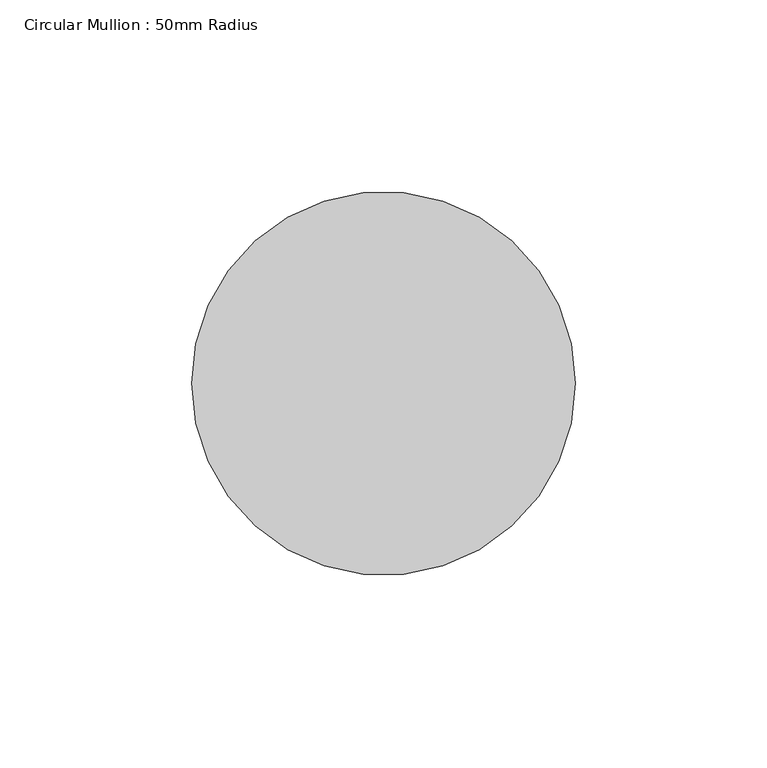
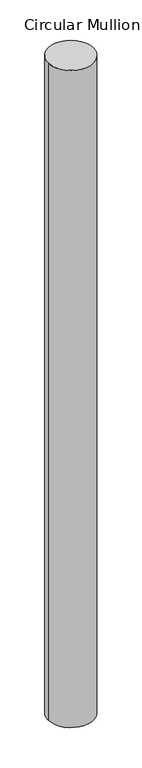
"""IFC4 building model written with IfcOpenShell, lengths in millimetres: member geometry, Circular Mullion : 50mm Radius."""

import ifcopenshell
import ifcopenshell.guid

model = None  # the IFC model being written
_history = None  # IfcOwnerHistory: only IFC2X3 demands one
_inside = {}  # id of a spatial element -> (the spatial element, [elements in it])
_under = {}  # id of a project, library or spatial element -> (it, [spatial elements below it])
_declared = {}  # id of a project -> (the project, [libraries it declares])
_typed = {}  # id of a type object -> (the type object, [elements of that type])
_made_of = {}  # id of a material, layer set ... -> (it, [elements and type objects made of it])


def new_model(schema):
    """Start an empty IFC model of exactly this schema.

    Asked for "IFC4X3", IfcOpenShell would pick the latest addendum, in which some entities
    have other attributes; the version numbers below select the first issue.
    IFC2X3 requires an IfcOwnerHistory on every rooted entity: one is made here for all.
    """
    global model, _history
    if schema == "IFC4X3":
        model = ifcopenshell.file(schema_version=(4, 3, 0, 0))
    else:
        model = ifcopenshell.file(schema=schema)
    _inside.clear()
    _under.clear()
    _declared.clear()
    _typed.clear()
    _made_of.clear()
    _history = None
    if model.schema == "IFC2X3":
        org = make("IfcOrganization", Name="unknown")
        user = make(
            "IfcPersonAndOrganization",
            ThePerson=make("IfcPerson", FamilyName="unknown"),
            TheOrganization=org,
        )
        app = make(
            "IfcApplication",
            ApplicationDeveloper=org,
            Version="unknown",
            ApplicationFullName="unknown",
            ApplicationIdentifier="unknown",
        )
        _history = make(
            "IfcOwnerHistory",
            OwningUser=user,
            OwningApplication=app,
            ChangeAction="ADDED",
            CreationDate=0,
        )
    return model


def make(cls, **values):
    """One entity of the class cls with the attributes given. An attribute that is None is left unset."""
    return model.create_entity(
        cls, **{name: value for name, value in values.items() if value is not None}
    )


def rooted(cls, **values):
    """An entity with a GlobalId (a new one), such as an element, a storey or a relation."""
    return make(cls, GlobalId=ifcopenshell.guid.new(), OwnerHistory=_history, **values)


def si_unit(unit_type, name, prefix=None):
    """IfcSIUnit, for example si_unit("LENGTHUNIT", "METRE", prefix="MILLI")."""
    return make("IfcSIUnit", UnitType=unit_type, Prefix=prefix, Name=name)


def assignment(units):
    """IfcUnitAssignment: the units of a project."""
    return None if units is None else make("IfcUnitAssignment", Units=units)


def point(xyz):
    """IfcCartesianPoint."""
    return None if xyz is None else make("IfcCartesianPoint", Coordinates=xyz)


def direction(xyz):
    """IfcDirection."""
    return None if xyz is None else make("IfcDirection", DirectionRatios=xyz)


def frame(location, z_axis=None, x_axis=None):
    """IfcAxis2Placement3D, a coordinate frame: its origin and axes. An axis left out is left unset."""
    return make(
        "IfcAxis2Placement3D",
        Location=point(location),
        Axis=direction(z_axis),
        RefDirection=direction(x_axis),
    )


def frame_2d(location, x_axis=None):
    """IfcAxis2Placement2D, a coordinate frame in the plane: its origin and x axis."""
    return make(
        "IfcAxis2Placement2D", Location=point(location), RefDirection=direction(x_axis)
    )


def origin():
    """The frame at (0, 0, 0) with its axes left unset."""
    return frame((0.0, 0.0, 0.0))


def origin_2d():
    """The frame at (0, 0) in the plane with its x axis left unset."""
    return frame_2d((0.0, 0.0))


def place(relative_to, where):
    """IfcLocalPlacement: puts the frame where relative to a parent placement (None: the world)."""
    return make(
        "IfcLocalPlacement", PlacementRelTo=relative_to, RelativePlacement=where
    )


def context(
    kind, dimensions, precision=None, world=None, true_north=None, identifier=None
):
    """IfcGeometricRepresentationContext, for example the 3D "Model" context."""
    return make(
        "IfcGeometricRepresentationContext",
        ContextIdentifier=identifier,
        ContextType=kind,
        CoordinateSpaceDimension=dimensions,
        Precision=precision,
        WorldCoordinateSystem=world,
        TrueNorth=true_north,
    )


def project(units=None, contexts=None):
    """IfcProject with its units and contexts."""
    return rooted(
        "IfcProject",
        Name="project",
        RepresentationContexts=contexts,
        UnitsInContext=assignment(units),
    )


def spatial(cls, under=None, at=None, **own):
    """A site, building, storey or space (cls), placed at a placement, below another one or the project."""
    s = rooted(cls, ObjectPlacement=at, **own)
    if under is not None:
        _under.setdefault(under.id(), (under, []))[1].append(s)
    return s


def circle_curve(where, radius):
    """IfcCircle in the frame where."""
    return make("IfcCircle", Position=where, Radius=radius)


def trimmed(basis, trim1, trim2, sense, master):
    """IfcTrimmedCurve: the piece of a basis curve between two trims."""
    return make(
        "IfcTrimmedCurve",
        BasisCurve=basis,
        Trim1=trim1,
        Trim2=trim2,
        SenseAgreement=sense,
        MasterRepresentation=master,
    )


def segment(curve, same_sense, transition):
    """IfcCompositeCurveSegment."""
    return make(
        "IfcCompositeCurveSegment",
        Transition=transition,
        SameSense=same_sense,
        ParentCurve=curve,
    )


def composite_curve(segments, self_intersect=None):
    """IfcCompositeCurve: segments joined end to end."""
    return make("IfcCompositeCurve", Segments=segments, SelfIntersect=self_intersect)


def outline(outer, holes=None, kind="AREA"):
    """IfcArbitraryClosedProfileDef: a profile drawn as a closed curve; with holes, ...WithVoids."""
    if holes is None:
        return make("IfcArbitraryClosedProfileDef", ProfileType=kind, OuterCurve=outer)
    return make(
        "IfcArbitraryProfileDefWithVoids",
        ProfileType=kind,
        OuterCurve=outer,
        InnerCurves=holes,
    )


def extrude(swept, where, along, depth):
    """IfcExtrudedAreaSolid: the profile swept, set in the frame where, extruded along a direction by depth."""
    return make(
        "IfcExtrudedAreaSolid",
        SweptArea=swept,
        Position=where,
        ExtrudedDirection=direction(along),
        Depth=depth,
    )


def shape(context_of_items, identifier, shape_type, items):
    """IfcShapeRepresentation: the items that make up one representation, for example the "Body"."""
    return make(
        "IfcShapeRepresentation",
        ContextOfItems=context_of_items,
        RepresentationIdentifier=identifier,
        RepresentationType=shape_type,
        Items=items,
    )


def source(mapping_origin, context_of_items, identifier, shape_type, items):
    """IfcRepresentationMap: a shape defined once, which mapped items show again and again."""
    return make(
        "IfcRepresentationMap",
        MappingOrigin=mapping_origin,
        MappedRepresentation=shape(context_of_items, identifier, shape_type, items),
    )


def transform(
    local_origin,
    x_axis=None,
    y_axis=None,
    z_axis=None,
    scale=None,
    scale2=None,
    scale3=None,
    uniform=True,
):
    """IfcCartesianTransformationOperator3D, or its non-uniform kind. x_axis, y_axis, z_axis: its Axis1, 2, 3."""
    if uniform:
        return make(
            "IfcCartesianTransformationOperator3D",
            Axis1=direction(x_axis),
            Axis2=direction(y_axis),
            LocalOrigin=point(local_origin),
            Scale=scale,
            Axis3=direction(z_axis),
        )
    return make(
        "IfcCartesianTransformationOperator3DnonUniform",
        Axis1=direction(x_axis),
        Axis2=direction(y_axis),
        LocalOrigin=point(local_origin),
        Scale=scale,
        Axis3=direction(z_axis),
        Scale2=scale2,
        Scale3=scale3,
    )


def mapped(mapping_source, mapping_target):
    """IfcMappedItem: shows the shape of a source again, moved by a transform."""
    return make(
        "IfcMappedItem", MappingSource=mapping_source, MappingTarget=mapping_target
    )


def made_of(thing, what):
    """Note that an element or type object is made of a material, layer set ...; save() writes the relation."""
    if what is not None:
        _made_of.setdefault(what.id(), (what, []))[1].append(thing)
    return thing


def element(
    cls,
    number,
    at=None,
    inside=None,
    cuts=None,
    type_object=None,
    material=None,
    context=None,
    identifier="Body",
    shape_type=None,
    held_by="IfcProductDefinitionShape",
    body=None,
    shapes=None,
    **own,
):
    """One element of the class cls, such as IfcWall. Its Tag is "e" and its number.

    at: its placement. inside: the storey or other place that contains it. cuts: it is an
    opening in that element (IfcRelVoidsElement). A single representation is given by context,
    identifier, shape_type and body (its items); several are given by shapes. held_by: the class
    of the entity that holds the representations. save() writes the other relations.
    """
    e = rooted(cls, Tag="e%d" % number, ObjectPlacement=at, **own)
    if body is not None:
        shapes = [shape(context, identifier, shape_type, body)]
    if shapes is not None:
        e.Representation = make(held_by, Representations=shapes)
    if inside is not None:
        _inside.setdefault(inside.id(), (inside, []))[1].append(e)
    if cuts is not None:
        rooted(
            "IfcRelVoidsElement", RelatingBuildingElement=cuts, RelatedOpeningElement=e
        )
    if type_object is not None:
        _typed.setdefault(type_object.id(), (type_object, []))[1].append(e)
    return made_of(e, material)


def aggregate(whole, parts):
    """IfcRelAggregates: a whole, such as a stair, and the parts it consists of."""
    return rooted("IfcRelAggregates", RelatingObject=whole, RelatedObjects=parts)


def save(model, path):
    """Write the relations noted so far, then the file.

    IfcRelAggregates (storeys below a building ...), IfcRelContainedInSpatialStructure (elements
    in a storey), IfcRelDefinesByType, IfcRelAssociatesMaterial and IfcRelDeclares: one each for
    every whole, place, type object, material and project.
    """
    for whole, parts in _under.values():
        aggregate(whole, parts)
    for where, things in _inside.values():
        rooted(
            "IfcRelContainedInSpatialStructure",
            RelatedElements=things,
            RelatingStructure=where,
        )
    for kind, things in _typed.values():
        rooted("IfcRelDefinesByType", RelatedObjects=things, RelatingType=kind)
    for what, things in _made_of.values():
        rooted("IfcRelAssociatesMaterial", RelatedObjects=things, RelatingMaterial=what)
    for by, libraries in _declared.values():
        rooted("IfcRelDeclares", RelatingContext=by, RelatedDefinitions=libraries)
    model.write(path)


def circular_mullion_50mm_radius_777ae902(model_context):
    return source(origin(), model_context, "Body", "SweptSolid", [
        extrude(outline(composite_curve([segment(trimmed(circle_curve(origin_2d(), 50.0), [point((50.0, 0.0))], [point((-50.0, 0.0))], False, "CARTESIAN"), True, "CONTINUOUS"), segment(trimmed(circle_curve(origin_2d(), 50.0), [point((-50.0, 0.0))], [point((50.0, 0.0))], False, "CARTESIAN"), True, "CONTINUOUS")], self_intersect=False)), frame((0.0, 0.0, -1528.2029638), z_axis=(0.0, 0.0, 1.0), x_axis=(1.0, 0.0, 0.0)), (0.0, 0.0, 1.0), 1528.2029638),
    ])


if __name__ == "__main__":
    model = new_model("IFC4")
    model_context = context("Model", 3, world=origin())
    ifc_project = project(units=[si_unit("LENGTHUNIT", "METRE", prefix="MILLI")], contexts=[model_context])
    site = spatial("IfcSite", under=ifc_project)
    building = spatial("IfcBuilding", under=site)
    placement = place(None, origin())
    circular_mullion_50mm_radius_shape = circular_mullion_50mm_radius_777ae902(model_context)
    element("IfcMember", 1, ObjectType="Circular Mullion : 50mm Radius", at=placement, inside=building, context=model_context, shape_type="MappedRepresentation", body=[
        mapped(circular_mullion_50mm_radius_shape, transform((0.0, 0.0, 0.0), x_axis=(1.0, 0.0, 0.0), y_axis=(0.0, 1.0, 0.0), z_axis=(0.0, 0.0, 1.0))),
    ])
    save(model, "model.ifc")

# Revit data of these elements
# Type "Circular Mullion : 50mm Radius"
#   built-in parameter 1007350 = 0.164042 (stored number, unit not read)
# Element 1 (IfcMember, "Circular Mullion : 50mm Radius")
#   Materials on its faces: "Aluminium"
# Materials
#   "Aluminium": class "Metal", colour RGB 247 247 247, transparency 0, Description = "Aluminium 6061", Cost = 0
